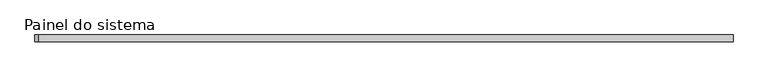
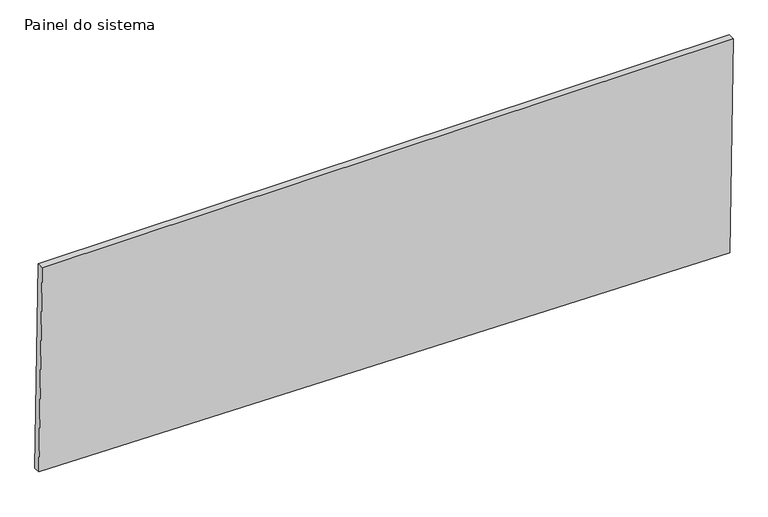
"""IFC4 building model written with IfcOpenShell, lengths in millimetres: plate geometry, Painel do sistema : Envidraçado."""

from ifc_helpers import new_model, si_unit, frame, origin, place, context, project, spatial, polyline, outline, extrude, source, transform, mapped, element, save


def painel_do_sistema_e261c9f3(model_context):
    return source(origin(), model_context, "Body", "SweptSolid", [
        extrude(outline(polyline([(37.9368749, -1267.3554827), (0.0, 1254.98818), (822.2761536, 1267.3554827), (822.2761536, -1255.5587631), (37.9368749, -1267.3554827)])), frame((0.0, 24.5, 0.0), z_axis=(0.0, 1.0, 0.0), x_axis=(0.0, 0.0, 1.0)), (0.0, 0.0, 1.0), 25.0),
    ])


if __name__ == "__main__":
    model = new_model("IFC4")
    model_context = context("Model", 3, world=origin())
    ifc_project = project(units=[si_unit("LENGTHUNIT", "METRE", prefix="MILLI")], contexts=[model_context])
    site = spatial("IfcSite", under=ifc_project)
    building = spatial("IfcBuilding", under=site)
    placement = place(None, origin())
    painel_do_sistema_shape = painel_do_sistema_e261c9f3(model_context)
    element("IfcPlate", 1, ObjectType="Painel do sistema : Envidraçado", at=placement, inside=building, context=model_context, shape_type="MappedRepresentation", body=[
        mapped(painel_do_sistema_shape, transform((0.0, 0.0, 0.0), x_axis=(1.0, 0.0, 0.0), y_axis=(0.0, 1.0, 0.0), z_axis=(0.0, 0.0, 1.0))),
    ])
    save(model, "model.ifc")

# Revit data of these elements
# Type "Painel do sistema : Envidraçado"
#   Construction Type Id = "GSP4R"
#   Analytic Construction = "Vidraça única Pilkington 1/8 pol"
#   Visual Light Transmittance = 0.9
#   Solar Heat Gain Coefficient = 0.86
#   Heat Transfer Coefficient (U) = 6.7069 W/(m²·K)
# Element 1 (IfcPlate, "Painel do sistema : Envidraçado")
#   Materials on its faces: "Vidro"
# Materials
#   "Vidro": class "Vidro", colour RGB 0 128 192, transparency 0.9, Description = "Vidro de sílica", Cost = 0
